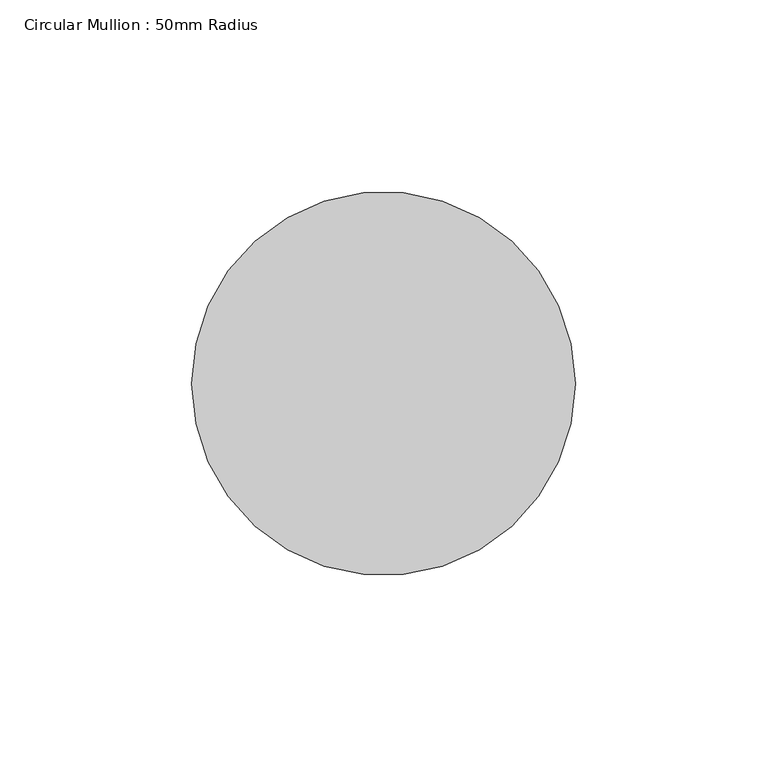
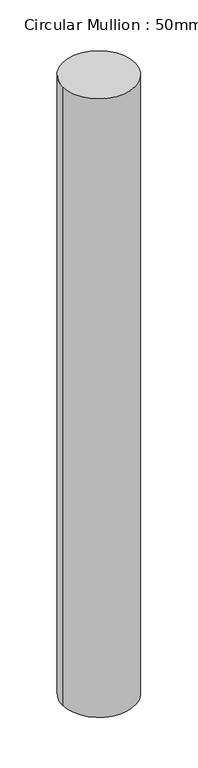
"""IFC4 building model written with IfcOpenShell, lengths in millimetres: member geometry, Circular Mullion : 50mm Radius."""

from ifc_helpers import new_model, si_unit, point, frame, origin, origin_2d, place, context, project, spatial, circle_curve, trimmed, segment, composite_curve, outline, extrude, source, transform, mapped, element, save


def circular_mullion_50mm_radius_3a98cae7(model_context):
    return source(origin(), model_context, "Body", "SweptSolid", [
        extrude(outline(composite_curve([segment(trimmed(circle_curve(origin_2d(), 50.0), [point((50.0, 0.0))], [point((-50.0, 0.0))], False, "CARTESIAN"), True, "CONTINUOUS"), segment(trimmed(circle_curve(origin_2d(), 50.0), [point((-50.0, 0.0))], [point((50.0, 0.0))], False, "CARTESIAN"), True, "CONTINUOUS")], self_intersect=False)), frame((0.0, 0.0, -901.7202279), z_axis=(0.0, 0.0, 1.0), x_axis=(1.0, 0.0, 0.0)), (0.0, 0.0, 1.0), 901.7202279),
    ])


if __name__ == "__main__":
    model = new_model("IFC4")
    model_context = context("Model", 3, world=origin())
    ifc_project = project(units=[si_unit("LENGTHUNIT", "METRE", prefix="MILLI")], contexts=[model_context])
    site = spatial("IfcSite", under=ifc_project)
    building = spatial("IfcBuilding", under=site)
    placement = place(None, origin())
    circular_mullion_50mm_radius_shape = circular_mullion_50mm_radius_3a98cae7(model_context)
    element("IfcMember", 1, ObjectType="Circular Mullion : 50mm Radius", at=placement, inside=building, context=model_context, shape_type="MappedRepresentation", body=[
        mapped(circular_mullion_50mm_radius_shape, transform((0.0, 0.0, 0.0), x_axis=(1.0, 0.0, 0.0), y_axis=(0.0, 1.0, 0.0), z_axis=(0.0, 0.0, 1.0))),
    ])
    save(model, "model.ifc")

# Revit data of these elements
# Type "Circular Mullion : 50mm Radius"
#   built-in parameter 1007350 = 0.164042 (stored number, unit not read)
# Element 1 (IfcMember, "Circular Mullion : 50mm Radius")
#   Materials on its faces: "Aluminium"
# Materials
#   "Aluminium": class "Metal", colour RGB 247 247 247, transparency 0, Description = "Aluminium 6061", Cost = 0
